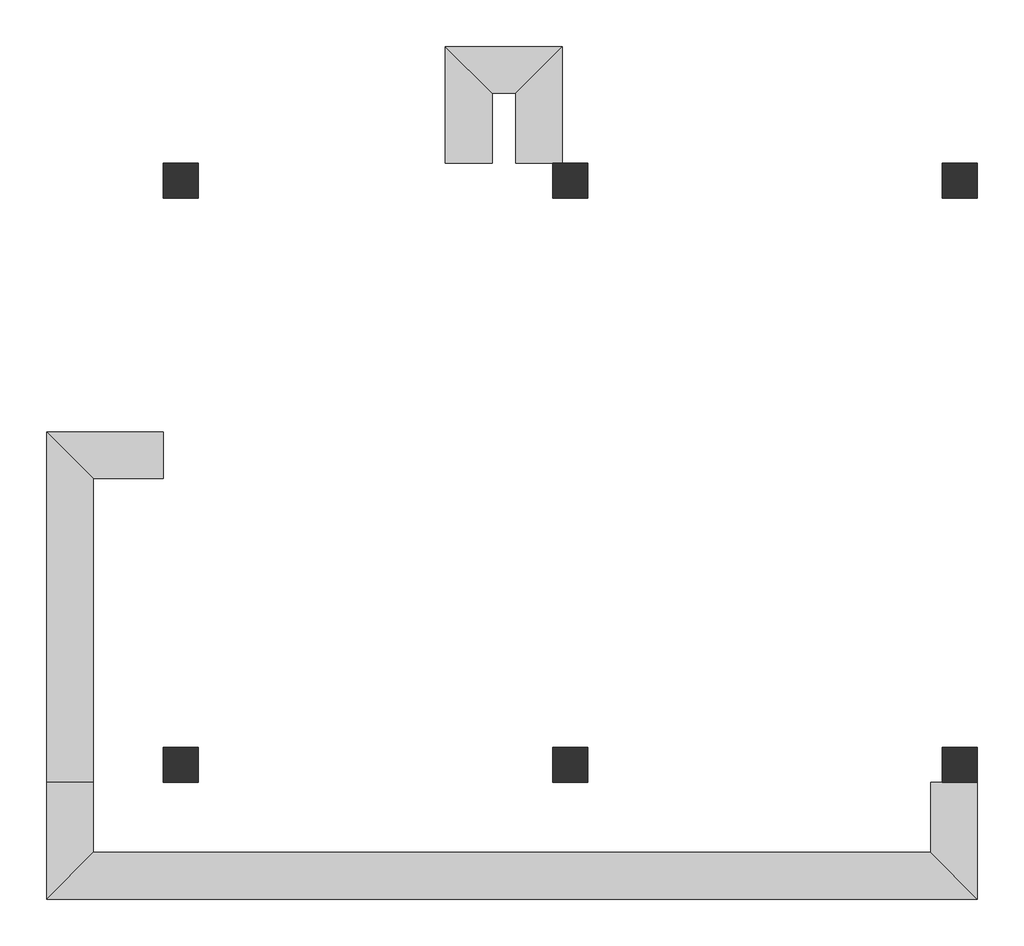
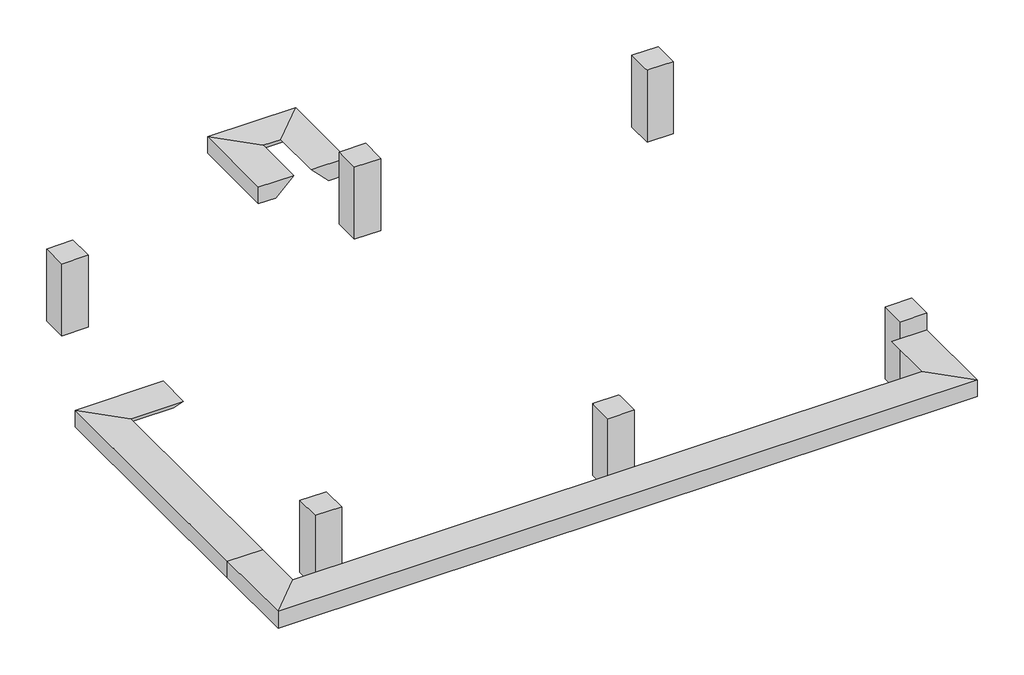
# One storey: 6 columns, 2 proxies.
"""IFC4 building model written with IfcOpenShell, lengths in millimetres."""

from ifc_helpers import new_model, si_unit, origin, place, context, project, spatial, faceted_brep, element, save

model = new_model("IFC4")

# Units and contexts
model_context = context("Model", 3, world=origin())
ifc_project = project(units=[si_unit("LENGTHUNIT", "METRE", prefix="MILLI")], contexts=[model_context])

# Site, building, storey
site = spatial("IfcSite", under=ifc_project)
building = spatial("IfcBuilding", under=site)
storey = spatial("IfcBuildingStorey", under=building, Name="T.O.C_-1,300", Elevation=-1300.0)

# Proxies
placement = place(None, origin())
element("IfcBuildingElementProxy", 1, Name="Slab Edge", ObjectType="Slab Edge", at=placement, inside=storey, context=model_context, shape_type="Brep", body=[
    faceted_brep([(4895.0, 21224.5208589, -450.0), (4895.0, 21224.5208589, -150.0), (4295.0, 21224.5208589, -150.0), (4595.0, 21224.5208589, -450.0), (4895.0, 22724.5208589, -450.0), (4895.0, 22724.5208589, -150.0), (4295.0, 22124.5208589, -150.0), (4595.0, 22424.5208589, -450.0), (3395.0, 22724.5208589, -450.0), (3395.0, 22724.5208589, -150.0), (3995.0, 22124.5208589, -150.0), (3695.0, 22424.5208589, -450.0), (3395.0, 21224.5208589, -450.0), (3695.0, 21224.5208589, -450.0), (3995.0, 21224.5208589, -150.0), (3395.0, 21224.5208589, -150.0)], [[[0, 1, 2, 3]], [[1, 0, 4, 5]], [[2, 1, 5, 6]], [[3, 2, 6, 7]], [[0, 3, 7, 4]], [[5, 4, 8, 9]], [[6, 5, 9, 10]], [[7, 6, 10, 11]], [[4, 7, 11, 8]], [[12, 13, 14, 15]], [[9, 8, 12, 15]], [[10, 9, 15, 14]], [[11, 10, 14, 13]], [[8, 11, 13, 12]]]),
])
element("IfcBuildingElementProxy", 2, Name="Slab Edge", ObjectType="Slab Edge", at=placement, inside=storey, context=model_context, shape_type="Brep", body=[
    faceted_brep([(10225.0, 13274.5208589, -600.0), (9925.0, 13274.5208589, -600.0), (9625.0, 13274.5208589, -300.0), (10225.0, 13274.5208589, -300.0), (10225.0, 11774.5208589, -300.0), (10225.0, 11774.5208589, -600.0), (9625.0, 12374.5208589, -300.0), (9925.0, 12074.5208589, -600.0), (-1725.0, 11774.5208589, -300.0), (-1725.0, 11774.5208589, -600.0), (-1125.0, 12374.5208589, -300.0), (-1425.0, 12074.5208589, -600.0), (-1725.0, 13274.5208589, -300.0), (-1725.0, 13274.5208589, -600.0), (-1125.0, 13274.5208589, -300.0), (-1425.0, 13274.5208589, -600.0), (-1725.0, 17774.5208589, -300.0), (-1725.0, 17774.5208589, -600.0), (-1125.0, 17174.5208589, -300.0), (-1425.0, 17474.5208589, -600.0), (-225.0, 17774.5208589, -600.0), (-225.0, 17774.5208589, -300.0), (-225.0, 17174.5208589, -300.0), (-225.0, 17474.5208589, -600.0)], [[[0, 1, 2, 3]], [[4, 5, 0, 3]], [[6, 4, 3, 2]], [[7, 6, 2, 1]], [[5, 7, 1, 0]], [[8, 9, 5, 4]], [[10, 8, 4, 6]], [[11, 10, 6, 7]], [[9, 11, 7, 5]], [[12, 13, 9, 8]], [[14, 12, 8, 10]], [[15, 14, 10, 11]], [[13, 15, 11, 9]], [[16, 17, 13, 12]], [[18, 16, 12, 14]], [[19, 18, 14, 15]], [[17, 19, 15, 13]], [[20, 21, 22, 23]], [[21, 20, 17, 16]], [[22, 21, 16, 18]], [[23, 22, 18, 19]], [[20, 23, 19, 17]]]),
])

# Columns
element("IfcColumn", 3, ObjectType="Concrete-Rectangular-Column : CL111_450x450", at=placement, inside=storey, context=model_context, shape_type="Brep", body=[
    faceted_brep([(225.0, 13724.5208589, -1300.0), (225.0, 13274.5208589, -1300.0), (-225.0, 13274.5208589, -1300.0), (-225.0, 13724.5208589, -1300.0), (225.0, 13724.5208589, 0.0), (225.0, 13674.5208589, 0.0), (225.0, 13274.5208589, 0.0), (225.0, 13274.5208589, -600.0), (-225.0, 13274.5208589, 0.0), (-225.0, 13724.5208589, 0.0), (-225.0, 13724.5208589, -600.0), (175.0, 13724.5208589, 0.0)], [[[0, 1, 2, 3]], [[4, 5, 6, 7, 1, 0]], [[6, 8, 2, 1, 7]], [[8, 9, 10, 3, 2]], [[9, 11, 4, 0, 3, 10]], [[4, 11, 9, 8, 6, 5]]]),
])
element("IfcColumn", 4, ObjectType="Concrete-Rectangular-Column : CL111_450x450", at=placement, inside=storey, context=model_context, shape_type="Brep", body=[
    faceted_brep([(5225.0, 13724.5208589, -1300.0), (5225.0, 13274.5208589, -1300.0), (4775.0, 13274.5208589, -1300.0), (4775.0, 13724.5208589, -1300.0), (5225.0, 13724.5208589, 0.0), (5225.0, 13674.5208589, 0.0), (5225.0, 13274.5208589, 0.0), (5225.0, 13274.5208589, -600.0), (4775.0, 13274.5208589, 0.0), (4775.0, 13274.5208589, -600.0), (4775.0, 13674.5208589, 0.0), (4775.0, 13724.5208589, 0.0)], [[[0, 1, 2, 3]], [[4, 5, 6, 7, 1, 0]], [[6, 8, 9, 2, 1, 7]], [[8, 10, 11, 3, 2, 9]], [[11, 4, 0, 3]], [[4, 11, 10, 8, 6, 5]]]),
])
element("IfcColumn", 5, ObjectType="Concrete-Rectangular-Column : CL111_450x450", at=placement, inside=storey, context=model_context, shape_type="Brep", body=[
    faceted_brep([(10225.0, 13724.5208589, -1300.0), (10225.0, 13274.5208589, -1300.0), (9775.0, 13274.5208589, -1300.0), (9775.0, 13724.5208589, -1300.0), (10225.0, 13724.5208589, 0.0), (10225.0, 13274.5208589, 0.0), (10225.0, 13724.5208589, -600.0), (9775.0, 13274.5208589, 0.0), (9775.0, 13274.5208589, -600.0), (9775.0, 13674.5208589, 0.0), (9775.0, 13724.5208589, 0.0), (9825.0, 13724.5208589, 0.0)], [[[0, 1, 2, 3]], [[4, 5, 1, 0, 6]], [[5, 7, 8, 2, 1]], [[7, 9, 10, 3, 2, 8]], [[10, 11, 4, 6, 0, 3]], [[4, 11, 10, 9, 7, 5]]]),
])
element("IfcColumn", 6, ObjectType="Concrete-Rectangular-Column : CL111_450x450", at=placement, inside=storey, context=model_context, shape_type="Brep", body=[
    faceted_brep([(10225.0, 21224.5208589, -1300.0), (10225.0, 20774.5208589, -1300.0), (9775.0, 20774.5208589, -1300.0), (9775.0, 21224.5208589, -1300.0), (10225.0, 21224.5208589, 0.0), (10225.0, 20774.5208589, 0.0), (10225.0, 20774.5208589, -600.0), (9825.0, 20774.5208589, 0.0), (9775.0, 20774.5208589, 0.0), (9775.0, 20834.5208589, 0.0), (9775.0, 21224.5208589, 0.0), (9775.0, 21224.5208589, -600.0)], [[[0, 1, 2, 3]], [[4, 5, 6, 1, 0]], [[5, 7, 8, 2, 1, 6]], [[8, 9, 10, 11, 3, 2]], [[10, 4, 0, 3, 11]], [[4, 10, 9, 8, 7, 5]]]),
])
element("IfcColumn", 7, ObjectType="Concrete-Rectangular-Column : CL111_450x450", at=placement, inside=storey, context=model_context, shape_type="Brep", body=[
    faceted_brep([(5225.0, 21224.5208589, -1300.0), (5225.0, 20774.5208589, -1300.0), (4775.0, 20774.5208589, -1300.0), (4775.0, 21224.5208589, -1300.0), (5225.0, 21224.5208589, 0.0), (5225.0, 20834.5208589, 0.0), (5225.0, 20774.5208589, 0.0), (5225.0, 21224.5208589, -600.0), (4775.0, 20774.5208589, 0.0), (4775.0, 21224.5208589, 0.0)], [[[0, 1, 2, 3]], [[4, 5, 6, 1, 0, 7]], [[6, 8, 2, 1]], [[8, 9, 3, 2]], [[9, 4, 7, 0, 3]], [[4, 9, 8, 6, 5]]]),
])
element("IfcColumn", 8, ObjectType="Concrete-Rectangular-Column : CL111_450x450", at=placement, inside=storey, context=model_context, shape_type="Brep", body=[
    faceted_brep([(225.0, 21224.5208589, -1300.0), (225.0, 20774.5208589, -1300.0), (-225.0, 20774.5208589, -1300.0), (-225.0, 21224.5208589, -1300.0), (225.0, 21224.5208589, 0.0), (225.0, 20834.5208589, 0.0), (225.0, 20774.5208589, 0.0), (225.0, 21224.5208589, -600.0), (175.0, 20774.5208589, 0.0), (-225.0, 20774.5208589, 0.0), (-225.0, 20774.5208589, -600.0), (-225.0, 21224.5208589, 0.0)], [[[0, 1, 2, 3]], [[4, 5, 6, 1, 0, 7]], [[6, 8, 9, 10, 2, 1]], [[9, 11, 3, 2, 10]], [[11, 4, 7, 0, 3]], [[4, 11, 9, 8, 6, 5]]]),
])

save(model, "model.ifc")

# Revit data of these elements
# Type "Concrete-Rectangular-Column : CL111_450x450"
#   Description = "UG 철골 기둥용 Pedestal"
#   b = 450 mm
#   h = 450 mm
#   hec_material3 [instance default] = none
#   hec_material2 [instance default] = A03AE056-00001_Bitumen/Bituminous/Asphalt Coating
#   hec_material1 [instance default] = A03AC035-00001_Form Work (3 times in use)_Flat
#   Structural Material [instance default] = A03AC032-00007_Structural Concrete_Type1_25MPa-30Mpa
# Element 1 (IfcBuildingElementProxy, "Slab Edge")
#   W11) Activity ID = "C02AGB040"
#   W12) Activity Name = "Main Gate Security Building ‐ Exterior & Finish Work"
#   W13) Plan Start Date = "2017-01-12"
#   W14) Plan Finish Date = "2017-04-11"
#   W15) Duration = "71"
#   W16) Actual Start Date = "2017-01-12"
#   W17) Actual Finish Date = "2017-04-11"
#   Phase Created = New Construction
#   Materials on its faces: "A03AD032-00007_Structural Concrete_25MPa-30MPa"
# Element 2 (IfcBuildingElementProxy, "Slab Edge")
#   Phase Created = New Construction
#   Materials on its faces: "A03AD032-00007_Structural Concrete_25MPa-30MPa"
# Elements 3, 4, 5, 6, 7, 8 (IfcColumn, "Concrete-Rectangular-Column : CL111_450x450")
#   Comments = ""
#   F01) Building Name = "Main Gate House"
#   F11) Project Building Tag_Type-1 = "Common"
#   F12) Project Building Tag_Type-2 = "Common"
#   F13) Project Facility Code = "Facility Code"
#   F21) Structural Type = "Concrete"
#   F31) Standard Building Code = "IBC"
#   F41) Discipline = "AR"
#   F51) Plan Start Date-Engineering = "2015-01-01"
#   F52) Plan Finish Date-Engineering = "2015-12-31"
#   F53) Duration = "365"
#   F54) Actual Start Date-Engineering = "2015-01-01"
#   F55) Actual Finish Date-Engineering = "2015-12-31"
#   F61) Plan Start Date-Construction = "2016-08-19"
#   F62) Plan Finish Date-Construction = "2017-01-31"
#   F64) Actual Start Date-Construction = "2016-08-19"
#   F63) Duration = "202"
#   F65) Actual Finish Date-Construction = "2017-01-31"
#   F91) Plant Type = "CFPP"
#   F92) KKS Structures, Building = "UYF"
#   P01) Project Name = "TVEP"
#   P02) Project Configuration = "CFB Boiler x 2(Foster Wheeler) + STG x 2(Alstom, 150MW)"
#   P03) Project Abbreviation = "TVEP"
#   P04) Project Code = "BEPH1402"
#   P05) Project Stage = "In operation"
#   P06) Project Location = "Sito Looc, Barangay Bato, Toledo City in Philippines"
#   P07) Project Owner = "Therma Visayas, Inc."
#   P08) Project O.E = "Flour"
#   P09) Project Schedule = "ITB Issueing Date : 2013.07.30\r\nSite Survey : 2013.08.19-20\r\nBid Closing Date : 2013.11.29\r\nPreferred Bidder Notice 접수 : 2014.04.27\r\nTarget award date : 2014 05\r\nLOA 접수 : 2014.05.21\r\nSigning Ceremony : 2014.05.30"
#   P10) Basic Wind Speed = "55.6 m/s"
#   P11) Seismic = "NSCP 2010, Zone 4 (PGA : 0.4g)"
#   P12) Soil = "Sc"
#   P13) Soil Capacity = "100kN/m2"
#   P14) Pile Capacity = "PHC(D400) : 1200kN"
#   W00) Work Master Code = "A03AC032-00007"
#   W01) Work Master_Lv1 = "Concrete Work"
#   W02) Work Master_Lv2 = "Substructure Work"
#   W03) Work Master_Spec.1 = "Structural Concrete"
#   W04) Work Master_Spec.2 = "Cement Type-1"
#   W05) Work Master_Spec.3 = "25MPa < F'c (Cylinder Strength) ≤ 30MPa"
#   W11) Activity ID = "C02AGB010"
#   W12) Activity Name = "Main Gate Security Building ‐ Building Foundaton"
#   W13) Plan Start Date = "2016-08-19"
#   W14) Plan Finish Date = "2016-09-22"
#   W15) Duration = "26"
#   W16) Actual Start Date = "2016-08-19"
#   W17) Actual Finish Date = "2016-09-22"
#   R02) Unit Price = 0
#   Structural Material = A03AD032-00007_Structural Concrete_25MPa-30MPa
#   hec_material3 = none
#   hec_material2 = none
#   hec_material1 = none
#   Phase Created = New Construction
#   Materials on its faces: "A03AD032-00007_Structural Concrete_25MPa-30MPa"
# Materials
#   "A03AE056-00001_Bitumen/Bituminous/Asphalt Coating": class "Generic", colour RGB 17 17 17, transparency 0, Description = "Damp-proofing", W00) Work Master Code = "A03AE056-00001", W01) Work Master_Lv1 = "Concrete Work", W02) Work Master_Lv2 = "Concrete Protective Coating (U/G)", W03) Work Master_Spec.1 = "Bitumen/Bituminous/Asphalt Coating", Cost = 0
#   "A03AC035-00001_Form Work (3 times in use)_Flat": class "Wood", colour RGB 149 120 74, transparency 0, Description = "Plywood", W00) Work Master Code = "A03AC035-00001", W01) Work Master_Lv1 = "Concrete Work", W02) Work Master_Lv2 = "Substructure Work", W03) Work Master_Spec.1 = "Form Work (3 times in use)", W04) Work Master_Spec.2 = "Flat Form", W05) Work Master_Spec.3 = "Dressed Lumber, Plywood or Steel Form(Wood Planks are not Allowed) incl. Chamfer", Cost = 0
#   "A03AC032-00007_Structural Concrete_Type1_25MPa-30Mpa": class "Concrete", colour RGB 176 176 176, transparency 0, Keynote = "09910.A1", Description = "Reinf. Conc.", W00) Work Master Code = "A03AC032-00007", W01) Work Master_Lv1 = "Concrete Work", W02) Work Master_Lv2 = "Substructure Work", W03) Work Master_Spec.1 = "Structural Concrete", W04) Work Master_Spec.2 = "Cement Type-1", W05) Work Master_Spec.3 = "25MPa < F'c (Cylinder Strength) ≤ 30MPa", Cost = 0
#   "A03AD032-00007_Structural Concrete_25MPa-30MPa": class "Concrete", colour RGB 176 176 176, transparency 0, Keynote = "09910.A1", Description = "Reinf. Conc.", W00) Work Master Code = "A03AD032-00007", W01) Work Master_Lv1 = "Concrete Work", W02) Work Master_Lv2 = "Superstructure Work", W03) Work Master_Spec.1 = "Structural Concrete", W04) Work Master_Spec.2 = "Cement Type-1", W05) Work Master_Spec.3 = "25MPa < F'c (Cylinder Strength) ≤ 30MPa", Cost = 0
# Room, not placed, phase "New Construction", upper offset 0 mm, lower offset 0 mm
#   Comments = ""
#   Base Finish = "EXPOXY PAINT ON THK.15 CEMENT PLASTER(H=100)"
#   Ceiling Finish = "LATEX PAINT ON FAIR FACED CONC."
#   Wall Finish = "LATEX PAINT ON THK.15 CEMENT PLASTER + MASONRY WALL"
#   Floor Finish = "EPOXY PAINT ON STEEL TROWELED CONC. SLAB"
#   Number = "1"
#   Name = ""
#   F01) Building Name = "CENTRAL CONTROL BUILDING"
#   S01) Room Name = "CABLE ROOM"
#   S02) Room Number(Project) = "UCA01R0001"
# Room, not placed, phase "New Construction", upper offset 0 mm, lower offset 0 mm
#   Comments = ""
#   Number = "2"
#   Name = ""
#   S01) Room Name = ""
#   S02) Room Number(Project) = ""
